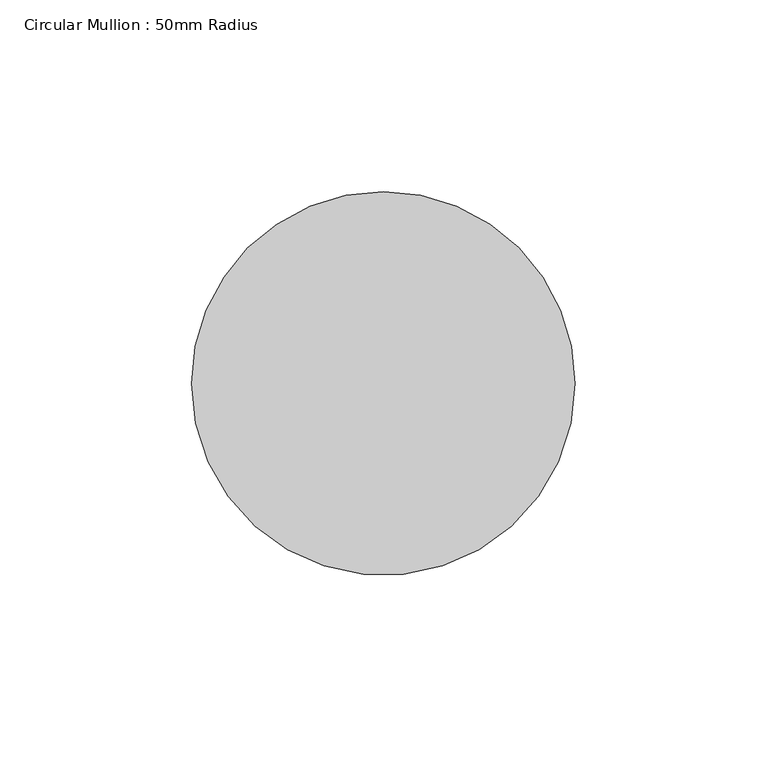
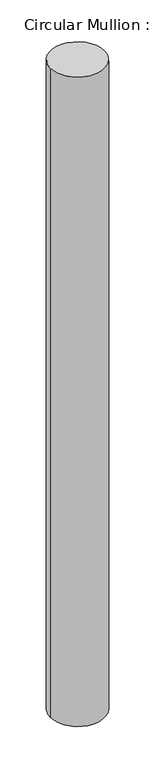
"""IFC4 building model written with IfcOpenShell, lengths in millimetres: member geometry, Circular Mullion : 50mm Radius."""

from ifc_helpers import new_model, si_unit, frame, origin, place, context, project, spatial, ellipse_curve, source, transform, mapped, element, save
from ifc_brep_helpers import plane_surface, cylinder_surface, advanced_brep


def circular_mullion_50mm_radius_13063f4d(model_context):
    return source(origin(), model_context, "Body", "AdvancedBrep", [
        advanced_brep(
        [(-100.0, 0.0, 0.3571079), (0.0, 0.0, 0.0), (0.0, 0.0, -1270.0250185), (-100.0, 0.0, -1270.6919508)],
        [
            (0, 1, ellipse_curve(frame((-50.0, 0.0, 0.1785539), z_axis=(-0.0035709693417899898, -0.006957025570452543, -0.9999694235191254), x_axis=(-0.4566331265276026, -0.8896207257763268, 0.00781997613986459)), 50.0015289, 50.0)),
            (1, 2),
            (2, 3, ellipse_curve(frame((-50.0, 0.0, -1270.3584847), z_axis=(-0.006668611607169479, -0.012991906966983092, 0.9998933643007109), x_axis=(0.4565983943069879, 0.8895530598502118, 0.014603425194313123)), 50.0053324, 50.0)),
            (3, 0),
            (1, 0, ellipse_curve(frame((-50.0, 0.0, 0.1785539), z_axis=(-0.0035709693417899898, -0.006957025570452543, -0.9999694235191254), x_axis=(-0.4566331265276026, -0.8896207257763268, 0.00781997613986459)), 50.0015289, 50.0)),
            (3, 2, ellipse_curve(frame((-50.0, 0.0, -1270.3584847), z_axis=(-0.006668611607169479, -0.012991906966983092, 0.9998933643007109), x_axis=(0.4565983943069879, 0.8895530598502118, 0.014603425194313123)), 50.0053324, 50.0)),
        ],
        [
            cylinder_surface(frame((-50.0, 0.0, 0.0), z_axis=(0.0, 0.0, 1.0), x_axis=(1.0, 0.0, 0.0)), 50.0),
            plane_surface(frame((-271.1646885, 139.1860328, 0.0), z_axis=(0.0035709693417899906, 0.006957025570452545, 0.9999694235191257), x_axis=(0.45663312652760474, 0.8896207257763259, -0.007819976139857115))),
            plane_surface(frame((-271.1646885, 139.1860328, -1270.0250185), z_axis=(0.006668611607169479, 0.012991906966983092, -0.9998933643007109), x_axis=(0.45659839430698784, 0.8895530598502117, 0.014603425194317232))),
        ],
        [
            (0, [[1, 2, 3, 4]]),
            (0, [[5, -4, 6, -2]]),
            (1, [[-1, -5]]),
            (2, [[-6, -3]]),
        ],
    ),
    ])


if __name__ == "__main__":
    model = new_model("IFC4")
    model_context = context("Model", 3, world=origin())
    ifc_project = project(units=[si_unit("LENGTHUNIT", "METRE", prefix="MILLI")], contexts=[model_context])
    site = spatial("IfcSite", under=ifc_project)
    building = spatial("IfcBuilding", under=site)
    placement = place(None, origin())
    circular_mullion_50mm_radius_shape = circular_mullion_50mm_radius_13063f4d(model_context)
    element("IfcMember", 1, ObjectType="Circular Mullion : 50mm Radius", at=placement, inside=building, context=model_context, shape_type="MappedRepresentation", body=[
        mapped(circular_mullion_50mm_radius_shape, transform((0.0, 0.0, 0.0), x_axis=(1.0, 0.0, 0.0), y_axis=(0.0, 1.0, 0.0), z_axis=(0.0, 0.0, 1.0))),
    ])
    save(model, "model.ifc")

# Revit data of these elements
# Type "Circular Mullion : 50mm Radius"
#   built-in parameter 1007350 = 0.164042 (stored number, unit not read)
# Element 1 (IfcMember, "Circular Mullion : 50mm Radius")
#   Materials on its faces: "Aluminium"
# Materials
#   "Aluminium": class "Metal", colour RGB 247 247 247, transparency 0, Description = "Aluminium 6061", Cost = 0
